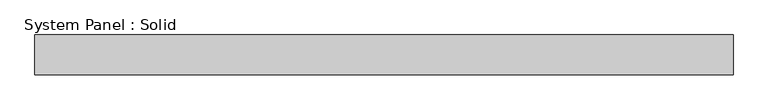
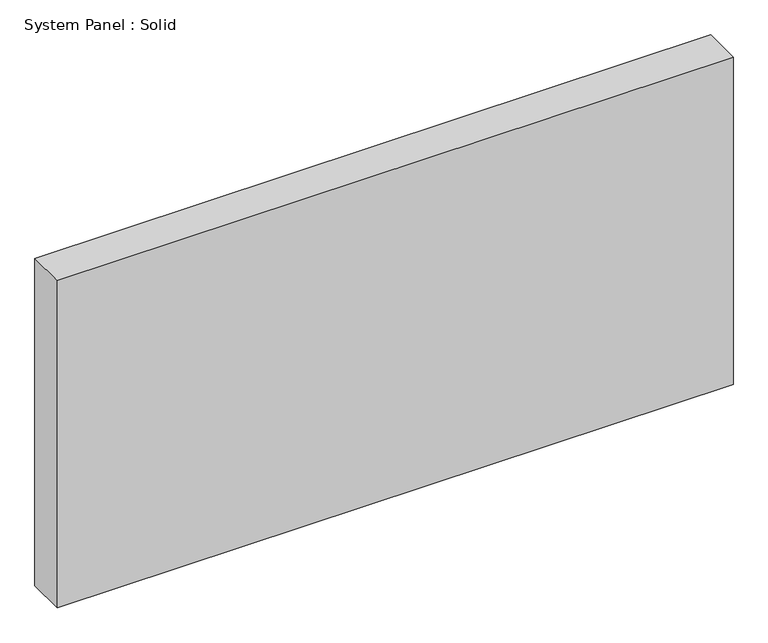
"""IFC4 building model written with IfcOpenShell, lengths in millimetres: plate geometry, System Panel : Solid."""

from ifc_helpers import new_model, si_unit, origin, origin_with_axes, place, context, project, spatial, polyline, outline, extrude, source, transform, mapped, element, save


def system_panel_solid_e4cae4a0(model_context):
    return source(origin(), model_context, "Body", "SweptSolid", [
        extrude(outline(polyline([(557.574914, -19.05), (-557.574914, -19.05), (-557.574914, 44.45), (557.574914, 44.45), (557.574914, -19.05)])), origin_with_axes(), (0.0, 0.0, 1.0), 571.5),
    ])


if __name__ == "__main__":
    model = new_model("IFC4")
    model_context = context("Model", 3, world=origin())
    ifc_project = project(units=[si_unit("LENGTHUNIT", "METRE", prefix="MILLI")], contexts=[model_context])
    site = spatial("IfcSite", under=ifc_project)
    building = spatial("IfcBuilding", under=site)
    placement = place(None, origin())
    system_panel_solid_shape = system_panel_solid_e4cae4a0(model_context)
    element("IfcPlate", 1, ObjectType="System Panel : Solid", at=placement, inside=building, context=model_context, shape_type="MappedRepresentation", body=[
        mapped(system_panel_solid_shape, transform((0.0, 0.0, 0.0), x_axis=(1.0, 0.0, 0.0), y_axis=(0.0, 1.0, 0.0), z_axis=(0.0, 0.0, 1.0))),
    ])
    save(model, "model.ifc")

# Revit data of these elements
# Element 1 (IfcPlate, "System Panel : Solid")
#   Materials on its faces: "Default"
# Materials
#   "Default": class "Miscellaneous", colour RGB 127 127 127, transparency 0
